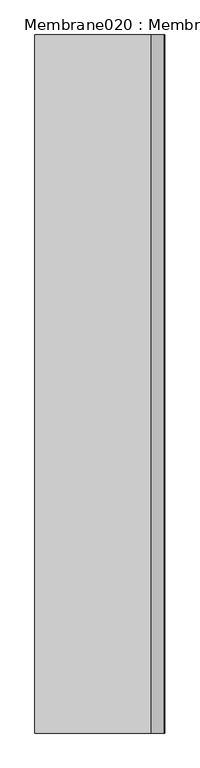
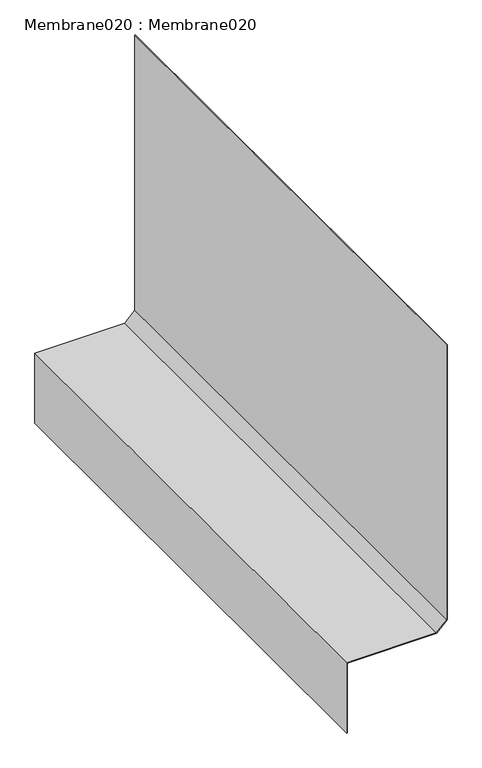
"""IFC4 building model written with IfcOpenShell, lengths in millimetres: proxy geometry, Membrane020 : Membrane020."""

from ifc_helpers import new_model, si_unit, frame, origin, place, context, project, spatial, polyline, outline, extrude, source, transform, mapped, element, save


def membrane020_membrane020_df872659(model_context):
    return source(origin(), model_context, "Body", "SweptSolid", [
        extrude(outline(polyline([(33706.6732458, -9667.8427734), (32628.5272919, -9667.8427734), (32590.4931641, -9705.461443), (32590.4931641, -10038.2705078), (32314.8961275, -10038.2705078), (32314.8961275, -10036.2705078), (32588.4931641, -10036.2705078), (32588.4931641, -9704.6265747), (32627.7052912, -9665.8427734), (33706.6732458, -9665.8427734), (33706.6732458, -9667.8427734)])), frame((0.0, 7182.1531721, 0.0), z_axis=(0.0, 1.0, 0.0), x_axis=(0.0, 0.0, 1.0)), (0.0, 0.0, 1.0), 2000.0),
    ])


if __name__ == "__main__":
    model = new_model("IFC4")
    model_context = context("Model", 3, world=origin())
    ifc_project = project(units=[si_unit("LENGTHUNIT", "METRE", prefix="MILLI")], contexts=[model_context])
    site = spatial("IfcSite", under=ifc_project)
    building = spatial("IfcBuilding", under=site)
    placement = place(None, origin())
    membrane020_membrane020_shape = membrane020_membrane020_df872659(model_context)
    element("IfcBuildingElementProxy", 1, Name="Membrane020 : Membrane020", ObjectType="Membrane020 : Membrane020", at=placement, inside=building, context=model_context, shape_type="MappedRepresentation", body=[
        mapped(membrane020_membrane020_shape, transform((0.0, 0.0, 0.0), x_axis=(1.0, 0.0, 0.0), y_axis=(0.0, 1.0, 0.0), z_axis=(0.0, 0.0, 1.0))),
    ])
    save(model, "model.ifc")

# Revit data of these elements
# Type "Membrane020 : Membrane020"
#   NameOverride = "Membrane020"
# Element 1 (IfcBuildingElementProxy, "Membrane020 : Membrane020")
#   Materials on its faces: "ECO ROOT BARRIER"
# Materials
#   "ECO ROOT BARRIER": class "Unassigned", colour RGB 135 255 2, transparency 0
